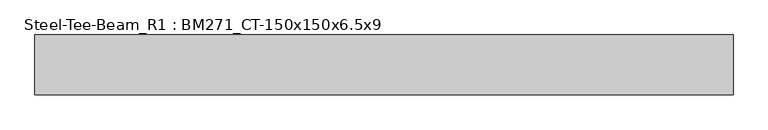
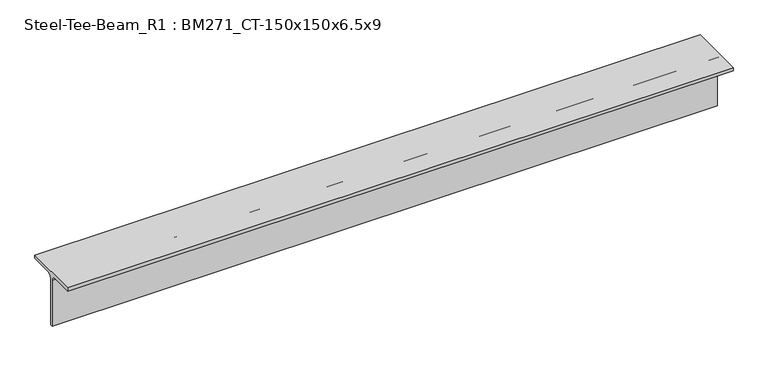
"""IFC4 building model written with IfcOpenShell, lengths in millimetres: member geometry, Steel-Tee-Beam_R1 : BM271_CT-150x150x6.5x9."""

from ifc_helpers import new_model, si_unit, point, frame, frame_2d, origin, place, context, project, spatial, polyline, circle_curve, trimmed, segment, composite_curve, outline, extrude, source, transform, mapped, element, save


def steel_tee_beam_r1_bm271_ct_150x150x6_5x9_cd676ca8(model_context):
    return source(origin(), model_context, "Body", "SweptSolid", [
        extrude(outline(composite_curve([segment(polyline([(-75.0, 75.0), (75.0, 75.0), (75.0, 66.0), (16.25, 66.0)]), True, "CONTINUOUS"), segment(trimmed(circle_curve(frame_2d((16.25, 53.0)), 13.0), [point((16.25, 66.0))], [point((3.25, 53.0))], True, "CARTESIAN"), True, "CONTINUOUS"), segment(polyline([(3.25, 53.0), (3.25, -75.0), (-3.25, -75.0), (-3.25, 53.0)]), True, "CONTINUOUS"), segment(trimmed(circle_curve(frame_2d((-16.25, 53.0)), 13.0), [point((-3.25, 53.0))], [point((-16.25, 66.0))], True, "CARTESIAN"), True, "CONTINUOUS"), segment(polyline([(-16.25, 66.0), (-75.0, 66.0), (-75.0, 75.0)]), True, "CONTINUOUS")], self_intersect=False)), frame((-983.9814396, 0.0, 0.0), z_axis=(1.0, 0.0, 0.0), x_axis=(0.0, 1.0, 0.0)), (0.0, 0.0, 1.0), 1754.8398202),
    ])


if __name__ == "__main__":
    model = new_model("IFC4")
    model_context = context("Model", 3, world=origin())
    ifc_project = project(units=[si_unit("LENGTHUNIT", "METRE", prefix="MILLI")], contexts=[model_context])
    site = spatial("IfcSite", under=ifc_project)
    building = spatial("IfcBuilding", under=site)
    placement = place(None, origin())
    steel_tee_beam_r1_bm271_ct_150x150x6_5x9_shape = steel_tee_beam_r1_bm271_ct_150x150x6_5x9_cd676ca8(model_context)
    element("IfcMember", 1, ObjectType="Steel-Tee-Beam_R1 : BM271_CT-150x150x6.5x9", at=placement, inside=building, context=model_context, shape_type="MappedRepresentation", body=[
        mapped(steel_tee_beam_r1_bm271_ct_150x150x6_5x9_shape, transform((0.0, 0.0, 0.0), x_axis=(1.0, 0.0, 0.0), y_axis=(0.0, 1.0, 0.0), z_axis=(0.0, 0.0, 1.0))),
    ])
    save(model, "model.ifc")

# Revit data of these elements
# Type "Steel-Tee-Beam_R1 : BM271_CT-150x150x6.5x9"
#   Keynote = "CT-150x150x6.5x9"
#   Surface Area = 0.588841 m²/m
#   Section Area = 23.3904 cm²
#   Mass per Unit Length = 18.3614 kg/m
#   Length [instance default] = 1.5240 m
#   bf = 0.1500 m
#   d = 0.1500 m
#   k = 0.0220 m
#   r = 0.0130 m
#   tf = 0.0090 m
#   tw = 0.0065 m
#   hec_material4 [instance default] = none
#   hec_material3 [instance default] = none
#   hec_material2 [instance default] = none
#   hec_material1 [instance default] = none
#   Structural Material [instance default] = Steel, 45-345
#   Assembly Code = ""
# Element 1 (IfcMember, "Steel-Tee-Beam_R1 : BM271_CT-150x150x6.5x9")
#   Structural Material = none
# Materials
#   "Steel, 45-345": class "Metal", colour RGB 189 187 185, transparency 0, Description = "Steel 345 MPa", Cost = 0
